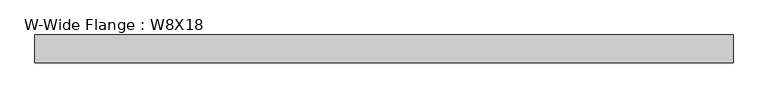
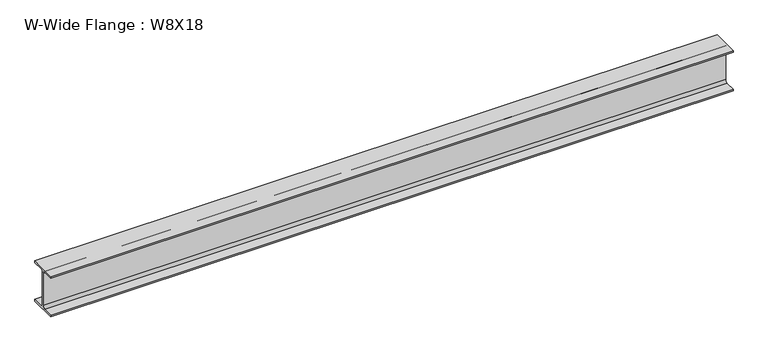
"""IFC4 building model written with IfcOpenShell, lengths in millimetres: beam geometry, W-Wide Flange : W8X18."""

import ifcopenshell
import ifcopenshell.guid

model = None  # the IFC model being written
_history = None  # IfcOwnerHistory: only IFC2X3 demands one
_inside = {}  # id of a spatial element -> (the spatial element, [elements in it])
_under = {}  # id of a project, library or spatial element -> (it, [spatial elements below it])
_declared = {}  # id of a project -> (the project, [libraries it declares])
_typed = {}  # id of a type object -> (the type object, [elements of that type])
_made_of = {}  # id of a material, layer set ... -> (it, [elements and type objects made of it])


def new_model(schema):
    """Start an empty IFC model of exactly this schema.

    Asked for "IFC4X3", IfcOpenShell would pick the latest addendum, in which some entities
    have other attributes; the version numbers below select the first issue.
    IFC2X3 requires an IfcOwnerHistory on every rooted entity: one is made here for all.
    """
    global model, _history
    if schema == "IFC4X3":
        model = ifcopenshell.file(schema_version=(4, 3, 0, 0))
    else:
        model = ifcopenshell.file(schema=schema)
    _inside.clear()
    _under.clear()
    _declared.clear()
    _typed.clear()
    _made_of.clear()
    _history = None
    if model.schema == "IFC2X3":
        org = make("IfcOrganization", Name="unknown")
        user = make(
            "IfcPersonAndOrganization",
            ThePerson=make("IfcPerson", FamilyName="unknown"),
            TheOrganization=org,
        )
        app = make(
            "IfcApplication",
            ApplicationDeveloper=org,
            Version="unknown",
            ApplicationFullName="unknown",
            ApplicationIdentifier="unknown",
        )
        _history = make(
            "IfcOwnerHistory",
            OwningUser=user,
            OwningApplication=app,
            ChangeAction="ADDED",
            CreationDate=0,
        )
    return model


def make(cls, **values):
    """One entity of the class cls with the attributes given. An attribute that is None is left unset."""
    return model.create_entity(
        cls, **{name: value for name, value in values.items() if value is not None}
    )


def rooted(cls, **values):
    """An entity with a GlobalId (a new one), such as an element, a storey or a relation."""
    return make(cls, GlobalId=ifcopenshell.guid.new(), OwnerHistory=_history, **values)


def si_unit(unit_type, name, prefix=None):
    """IfcSIUnit, for example si_unit("LENGTHUNIT", "METRE", prefix="MILLI")."""
    return make("IfcSIUnit", UnitType=unit_type, Prefix=prefix, Name=name)


def assignment(units):
    """IfcUnitAssignment: the units of a project."""
    return None if units is None else make("IfcUnitAssignment", Units=units)


def point(xyz):
    """IfcCartesianPoint."""
    return None if xyz is None else make("IfcCartesianPoint", Coordinates=xyz)


def direction(xyz):
    """IfcDirection."""
    return None if xyz is None else make("IfcDirection", DirectionRatios=xyz)


def frame(location, z_axis=None, x_axis=None):
    """IfcAxis2Placement3D, a coordinate frame: its origin and axes. An axis left out is left unset."""
    return make(
        "IfcAxis2Placement3D",
        Location=point(location),
        Axis=direction(z_axis),
        RefDirection=direction(x_axis),
    )


def frame_2d(location, x_axis=None):
    """IfcAxis2Placement2D, a coordinate frame in the plane: its origin and x axis."""
    return make(
        "IfcAxis2Placement2D", Location=point(location), RefDirection=direction(x_axis)
    )


def origin():
    """The frame at (0, 0, 0) with its axes left unset."""
    return frame((0.0, 0.0, 0.0))


def place(relative_to, where):
    """IfcLocalPlacement: puts the frame where relative to a parent placement (None: the world)."""
    return make(
        "IfcLocalPlacement", PlacementRelTo=relative_to, RelativePlacement=where
    )


def context(
    kind, dimensions, precision=None, world=None, true_north=None, identifier=None
):
    """IfcGeometricRepresentationContext, for example the 3D "Model" context."""
    return make(
        "IfcGeometricRepresentationContext",
        ContextIdentifier=identifier,
        ContextType=kind,
        CoordinateSpaceDimension=dimensions,
        Precision=precision,
        WorldCoordinateSystem=world,
        TrueNorth=true_north,
    )


def project(units=None, contexts=None):
    """IfcProject with its units and contexts."""
    return rooted(
        "IfcProject",
        Name="project",
        RepresentationContexts=contexts,
        UnitsInContext=assignment(units),
    )


def spatial(cls, under=None, at=None, **own):
    """A site, building, storey or space (cls), placed at a placement, below another one or the project."""
    s = rooted(cls, ObjectPlacement=at, **own)
    if under is not None:
        _under.setdefault(under.id(), (under, []))[1].append(s)
    return s


def polyline(points):
    """IfcPolyline through the points."""
    return make("IfcPolyline", Points=[point(p) for p in points])


def circle_curve(where, radius):
    """IfcCircle in the frame where."""
    return make("IfcCircle", Position=where, Radius=radius)


def trimmed(basis, trim1, trim2, sense, master):
    """IfcTrimmedCurve: the piece of a basis curve between two trims."""
    return make(
        "IfcTrimmedCurve",
        BasisCurve=basis,
        Trim1=trim1,
        Trim2=trim2,
        SenseAgreement=sense,
        MasterRepresentation=master,
    )


def segment(curve, same_sense, transition):
    """IfcCompositeCurveSegment."""
    return make(
        "IfcCompositeCurveSegment",
        Transition=transition,
        SameSense=same_sense,
        ParentCurve=curve,
    )


def composite_curve(segments, self_intersect=None):
    """IfcCompositeCurve: segments joined end to end."""
    return make("IfcCompositeCurve", Segments=segments, SelfIntersect=self_intersect)


def outline(outer, holes=None, kind="AREA"):
    """IfcArbitraryClosedProfileDef: a profile drawn as a closed curve; with holes, ...WithVoids."""
    if holes is None:
        return make("IfcArbitraryClosedProfileDef", ProfileType=kind, OuterCurve=outer)
    return make(
        "IfcArbitraryProfileDefWithVoids",
        ProfileType=kind,
        OuterCurve=outer,
        InnerCurves=holes,
    )


def extrude(swept, where, along, depth):
    """IfcExtrudedAreaSolid: the profile swept, set in the frame where, extruded along a direction by depth."""
    return make(
        "IfcExtrudedAreaSolid",
        SweptArea=swept,
        Position=where,
        ExtrudedDirection=direction(along),
        Depth=depth,
    )


def shape(context_of_items, identifier, shape_type, items):
    """IfcShapeRepresentation: the items that make up one representation, for example the "Body"."""
    return make(
        "IfcShapeRepresentation",
        ContextOfItems=context_of_items,
        RepresentationIdentifier=identifier,
        RepresentationType=shape_type,
        Items=items,
    )


def source(mapping_origin, context_of_items, identifier, shape_type, items):
    """IfcRepresentationMap: a shape defined once, which mapped items show again and again."""
    return make(
        "IfcRepresentationMap",
        MappingOrigin=mapping_origin,
        MappedRepresentation=shape(context_of_items, identifier, shape_type, items),
    )


def transform(
    local_origin,
    x_axis=None,
    y_axis=None,
    z_axis=None,
    scale=None,
    scale2=None,
    scale3=None,
    uniform=True,
):
    """IfcCartesianTransformationOperator3D, or its non-uniform kind. x_axis, y_axis, z_axis: its Axis1, 2, 3."""
    if uniform:
        return make(
            "IfcCartesianTransformationOperator3D",
            Axis1=direction(x_axis),
            Axis2=direction(y_axis),
            LocalOrigin=point(local_origin),
            Scale=scale,
            Axis3=direction(z_axis),
        )
    return make(
        "IfcCartesianTransformationOperator3DnonUniform",
        Axis1=direction(x_axis),
        Axis2=direction(y_axis),
        LocalOrigin=point(local_origin),
        Scale=scale,
        Axis3=direction(z_axis),
        Scale2=scale2,
        Scale3=scale3,
    )


def mapped(mapping_source, mapping_target):
    """IfcMappedItem: shows the shape of a source again, moved by a transform."""
    return make(
        "IfcMappedItem", MappingSource=mapping_source, MappingTarget=mapping_target
    )


def made_of(thing, what):
    """Note that an element or type object is made of a material, layer set ...; save() writes the relation."""
    if what is not None:
        _made_of.setdefault(what.id(), (what, []))[1].append(thing)
    return thing


def element(
    cls,
    number,
    at=None,
    inside=None,
    cuts=None,
    type_object=None,
    material=None,
    context=None,
    identifier="Body",
    shape_type=None,
    held_by="IfcProductDefinitionShape",
    body=None,
    shapes=None,
    **own,
):
    """One element of the class cls, such as IfcWall. Its Tag is "e" and its number.

    at: its placement. inside: the storey or other place that contains it. cuts: it is an
    opening in that element (IfcRelVoidsElement). A single representation is given by context,
    identifier, shape_type and body (its items); several are given by shapes. held_by: the class
    of the entity that holds the representations. save() writes the other relations.
    """
    e = rooted(cls, Tag="e%d" % number, ObjectPlacement=at, **own)
    if body is not None:
        shapes = [shape(context, identifier, shape_type, body)]
    if shapes is not None:
        e.Representation = make(held_by, Representations=shapes)
    if inside is not None:
        _inside.setdefault(inside.id(), (inside, []))[1].append(e)
    if cuts is not None:
        rooted(
            "IfcRelVoidsElement", RelatingBuildingElement=cuts, RelatedOpeningElement=e
        )
    if type_object is not None:
        _typed.setdefault(type_object.id(), (type_object, []))[1].append(e)
    return made_of(e, material)


def aggregate(whole, parts):
    """IfcRelAggregates: a whole, such as a stair, and the parts it consists of."""
    return rooted("IfcRelAggregates", RelatingObject=whole, RelatedObjects=parts)


def save(model, path):
    """Write the relations noted so far, then the file.

    IfcRelAggregates (storeys below a building ...), IfcRelContainedInSpatialStructure (elements
    in a storey), IfcRelDefinesByType, IfcRelAssociatesMaterial and IfcRelDeclares: one each for
    every whole, place, type object, material and project.
    """
    for whole, parts in _under.values():
        aggregate(whole, parts)
    for where, things in _inside.values():
        rooted(
            "IfcRelContainedInSpatialStructure",
            RelatedElements=things,
            RelatingStructure=where,
        )
    for kind, things in _typed.values():
        rooted("IfcRelDefinesByType", RelatedObjects=things, RelatingType=kind)
    for what, things in _made_of.values():
        rooted("IfcRelAssociatesMaterial", RelatedObjects=things, RelatingMaterial=what)
    for by, libraries in _declared.values():
        rooted("IfcRelDeclares", RelatingContext=by, RelatedDefinitions=libraries)
    model.write(path)


def w_wide_flange_w8x18_57e2a91b(model_context):
    return source(origin(), model_context, "Body", "SweptSolid", [
        extrude(outline(composite_curve([segment(polyline([(66.675, -94.996), (66.675, -103.378), (-66.675, -103.378), (-66.675, -94.996), (-15.1765, -94.996)]), True, "CONTINUOUS"), segment(trimmed(circle_curve(frame_2d((-15.1765, -82.7405)), 12.2555), [point((-15.1765, -94.996))], [point((-2.921, -82.7405))], True, "CARTESIAN"), True, "CONTINUOUS"), segment(polyline([(-2.921, -82.7405), (-2.921, 82.7405)]), True, "CONTINUOUS"), segment(trimmed(circle_curve(frame_2d((-15.1765, 82.7405)), 12.2555), [point((-2.921, 82.7405))], [point((-15.1765, 94.996))], True, "CARTESIAN"), True, "CONTINUOUS"), segment(polyline([(-15.1765, 94.996), (-66.675, 94.996), (-66.675, 103.378), (66.675, 103.378), (66.675, 94.996), (15.1765, 94.996)]), True, "CONTINUOUS"), segment(trimmed(circle_curve(frame_2d((15.1765, 82.7405)), 12.2555), [point((15.1765, 94.996))], [point((2.921, 82.7405))], True, "CARTESIAN"), True, "CONTINUOUS"), segment(polyline([(2.921, 82.7405), (2.921, -82.7405)]), True, "CONTINUOUS"), segment(trimmed(circle_curve(frame_2d((15.1765, -82.7405)), 12.2555), [point((2.921, -82.7405))], [point((15.1765, -94.996))], True, "CARTESIAN"), True, "CONTINUOUS"), segment(polyline([(15.1765, -94.996), (66.675, -94.996)]), True, "CONTINUOUS")], self_intersect=False)), frame((-1658.9375, 0.0, 0.0), z_axis=(1.0, 0.0, 0.0), x_axis=(0.0, 1.0, 0.0)), (0.0, 0.0, 1.0), 3317.875),
    ])


if __name__ == "__main__":
    model = new_model("IFC4")
    model_context = context("Model", 3, world=origin())
    ifc_project = project(units=[si_unit("LENGTHUNIT", "METRE", prefix="MILLI")], contexts=[model_context])
    site = spatial("IfcSite", under=ifc_project)
    building = spatial("IfcBuilding", under=site)
    placement = place(None, origin())
    w_wide_flange_w8x18_shape = w_wide_flange_w8x18_57e2a91b(model_context)
    element("IfcBeam", 1, ObjectType="W-Wide Flange : W8X18", at=placement, inside=building, context=model_context, shape_type="MappedRepresentation", body=[
        mapped(w_wide_flange_w8x18_shape, transform((0.0, 0.0, 0.0), x_axis=(1.0, 0.0, 0.0), y_axis=(0.0, 1.0, 0.0), z_axis=(0.0, 0.0, 1.0))),
    ])
    save(model, "model.ifc")

# Revit data of these elements
# Type "W-Wide Flange : W8X18"
#   Assembly Code = "B10"
#   W = 18
#   Length [instance default] = 1524 mm
#   bf = 133.35 mm
#   d = 206.756 mm
#   k = 20.638 mm
#   k2 = 12.256 mm
#   tf = 8.382 mm
#   tw = 5.842 mm
#   A = 0.00339354 m²
#   Structural Material [instance default] = Steel ASTM A992
# Element 1 (IfcBeam, "W-Wide Flange : W8X18")
#   Structural Material = Aluminum, Anodized Red
#   Materials on its faces: "Aluminum, Anodized Red"
# Materials
#   "Steel ASTM A992": class "Metal", colour RGB 128 0 0, transparency 0, Description = "Structural steel 50ksi", Cost = 0
#   "Aluminum, Anodized Red": class "Metal", colour RGB 120 120 120, transparency 0, Description = "Anodized aluminum, red", Cost = 0
